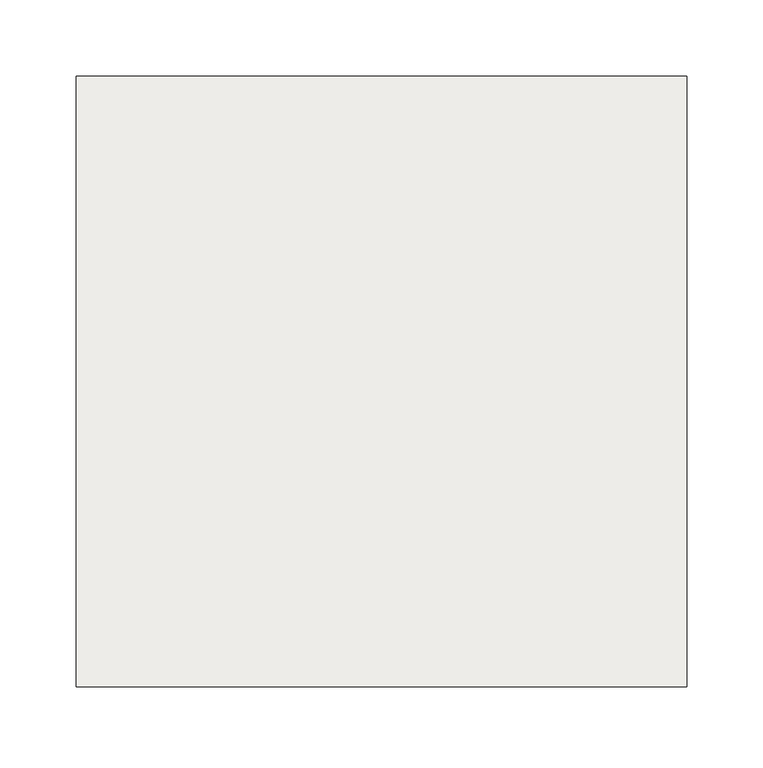
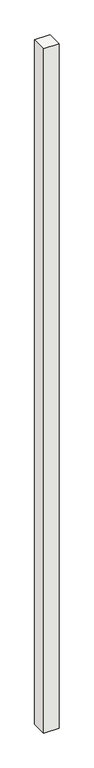
"""IFC4 building model written with IfcOpenShell, lengths in millimetres: slab geometry, NLRS_17_SFO_TLB_funderingspaal geheid beton prefab-AV-MMBPC_gen_rsf : heipaal beton prefab_gen__bxh 400x400."""

from ifc_helpers import new_model, si_unit, frame, origin, place, context, project, spatial, polyline, outline, extrude, source, transform, mapped, element, save


def slab_0d914d5e(model_context):
    return source(origin(), model_context, "Body", "SweptSolid", [
        extrude(outline(polyline([(200.0, -200.0), (-200.0, -200.0), (-200.0, 200.0), (200.0, 200.0), (200.0, -200.0)])), frame((0.0, 0.0, -20000.0), z_axis=(0.0, 0.0, 1.0), x_axis=(1.0, 0.0, 0.0)), (0.0, 0.0, 1.0), 18850.0),
    ])


if __name__ == "__main__":
    model = new_model("IFC4")
    model_context = context("Model", 3, world=origin())
    ifc_project = project(units=[si_unit("LENGTHUNIT", "METRE", prefix="MILLI")], contexts=[model_context])
    site = spatial("IfcSite", under=ifc_project)
    building = spatial("IfcBuilding", under=site)
    placement = place(None, origin())
    slab_shape = slab_0d914d5e(model_context)
    element("IfcSlab", 1, ObjectType="NLRS_17_SFO_TLB_funderingspaal geheid beton prefab-AV-MMBPC_gen_rsf : heipaal beton prefab_gen__bxh 400x400", at=placement, inside=building, context=model_context, shape_type="MappedRepresentation", body=[
        mapped(slab_shape, transform((0.0, 0.0, 0.0), x_axis=(1.0, 0.0, 0.0), y_axis=(0.0, 1.0, 0.0), z_axis=(0.0, 0.0, 1.0))),
    ])
    save(model, "model.ifc")

# Revit data of these elements
# Type "NLRS_17_SFO_TLB_funderingspaal geheid beton prefab-AV-MMBPC_gen_rsf : heipaal beton prefab_gen__bxh 400x400"
#   Export Type to IFC As = "IfcPile"
#   Type IfcGUID = "10$Kfo5uPCAOPJEOo5LE_W"
#   Type Comments = "prefab heipaal 400x400"
#   Model = " "
#   Manufacturer = " "
#   Description = "prefab heipaal 400x400"
#   Assembly Code = "17.21"
#   Width = 400 mm
#   Slanted Angle [instance default] = 0.00°
#   NLRS_S_draagvermogen_trek [instance default] = 0.00 kN
#   NLRS_S_draagvermogen_druk [instance default] = 0.00 kN
#   NLRS_C_lengte [instance default] = 1660 mm
#   NLRS_C_hoogte = 400 mm
#   NLRS_C_breedte = 400 mm
#   Height [instance default] = 1660 mm
#   Length [instance default] = 1660 mm
#   Angle [instance default] = 0.00°
#   Slanted [instance default] = 0
#   Structural Material = NLRS_f2_beton prefab_gen_rsf
#   Keynote = ""
# Element 1 (IfcSlab, "NLRS_17_SFO_TLB_funderingspaal geheid beton prefab-AV-MMBPC_gen_rsf : heipaal beton prefab_gen__bxh 400x400")
#   NLRS_C_lengte = 18850 mm
#   Height = 18850 mm
#   Length = 18850 mm
#   Materials on its faces: "NLRS_f2_beton prefab_gen_rsf"
# Materials
#   "NLRS_f2_beton prefab_gen_rsf": class "F - Niet gebakken kunststeen", colour RGB 129 133 118, transparency 0, Keynote = "f2", Manufacturer = "Revit Standards Foundation", URL = "www.revitstandards.org", Description = "beton prefab", Cost = 0
